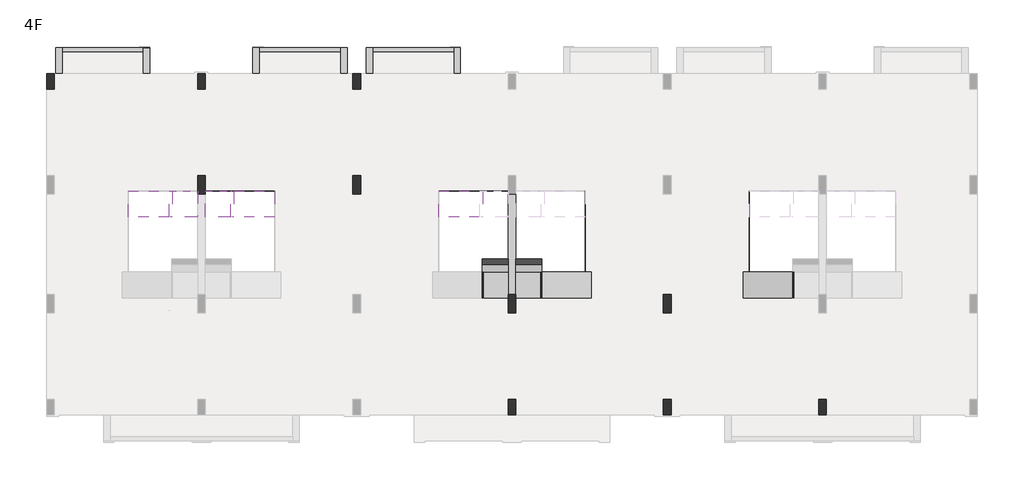
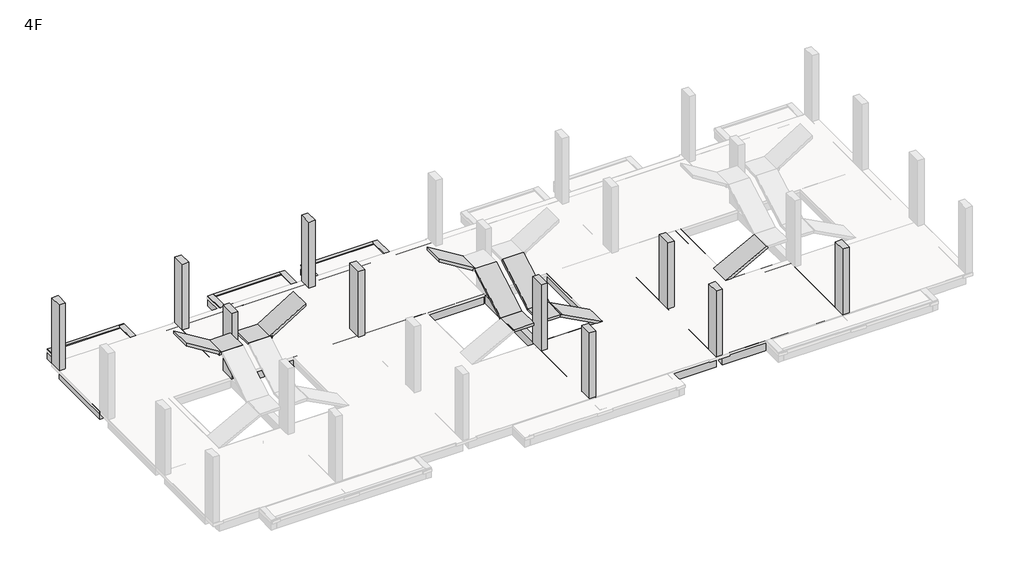
# One storey, part 2 of 3: 39 beams, 10 columns.
"""IFC4 building model written with IfcOpenShell, lengths in millimetres."""

from ifc_helpers import new_model, si_unit, frame, origin, place, context, project, spatial, polyline, outline, extrude, faceted_brep, element, save

model = new_model("IFC4")

# Units and contexts
model_context = context("Model", 3, world=origin())
ifc_project = project(units=[si_unit("LENGTHUNIT", "METRE", prefix="MILLI")], contexts=[model_context])

# Site, building, storey
site = spatial("IfcSite", under=ifc_project)
building = spatial("IfcBuilding", under=site)
storey = spatial("IfcBuildingStorey", under=building, Name="4F", Elevation=10630.0)

# Beams
placement = place(None, origin())
element("IfcBeam", 1, ObjectType="M_Concrete-Rectangular Beam : 1000x120", at=placement, inside=storey, context=model_context, shape_type="Brep", body=[
    faceted_brep([(4600.0000007, 7550.0000002, 12880.0), (4600.0000007, 8550.0000002, 12880.0), (4600.0000007, 8550.0000002, 12760.0), (4600.0000007, 7550.0000002, 12760.0), (5700.0000007, 8550.0000002, 12760.0), (5700.0000007, 8550.0000002, 12880.0), (5700.0000007, 7550.0000002, 12880.0), (5700.0000007, 7609.0063595, 12775.5095719), (5700.0000007, 7581.5414925, 12760.0), (4700.0000007, 7550.0000002, 12880.0), (4700.0000007, 7581.5414925, 12760.0), (4700.0000007, 7550.0000002, 12760.0), (4700.0000007, 7609.0063595, 12775.5095719)], [[[0, 1, 2, 3]], [[4, 5, 6, 7, 8]], [[1, 0, 9, 6, 5]], [[2, 1, 5, 4]], [[3, 2, 4, 8, 10, 11]], [[0, 3, 11, 9]], [[12, 7, 6, 9]], [[7, 12, 10, 8]], [[12, 9, 11, 10]]]),
])
element("IfcBeam", 2, ObjectType="M_Concrete-Rectangular Beam : 1000x120", at=placement, inside=storey, context=model_context, shape_type="Brep", body=[
    faceted_brep([(3019.99996, 7549.9999993, 13930.0), (4715.7503089, 7549.9999993, 12880.0), (4715.7503089, 8549.9999993, 12880.0), (3019.99996, 8549.9999993, 13930.0), (4600.0000007, 8549.9999993, 12880.0), (4600.0000007, 8549.9999993, 12810.5302519), (3020.0, 8549.9999993, 13788.8582245), (4600.0000007, 7549.9999993, 12810.5302519), (3020.0, 7549.9999993, 13788.8582245), (4600.0000007, 7549.9999993, 12880.0), (4700.0000007, 7549.9999993, 12880.0)], [[[0, 1, 2, 3]], [[3, 2, 4, 5, 6]], [[5, 7, 8, 6]], [[1, 0, 8, 7, 9, 10]], [[4, 9, 7, 5]], [[9, 4, 2, 1, 10]], [[0, 3, 6, 8]]]),
])
element("IfcBeam", 3, ObjectType="M_Concrete-Rectangular Beam : 1000x120", at=placement, inside=storey, context=model_context, shape_type="Brep", body=[
    faceted_brep([(7100.0000007, 8550.0000002, 12880.0), (7100.0000007, 7550.0000002, 12880.0), (7100.0000007, 7550.0000002, 12760.0), (7100.0000007, 8550.0000002, 12760.0), (6000.0000007, 8550.0000002, 12880.0), (6000.0000007, 8550.0000002, 12760.0), (6000.0000007, 7581.5414925, 12760.0), (6000.0000007, 7609.0063595, 12775.5095719), (6000.0000007, 7550.0000002, 12880.0), (7000.0000007, 7550.0000002, 12880.0), (7000.0000007, 7550.0000002, 12760.0), (7000.0000007, 7581.5414925, 12760.0), (7000.0000007, 7609.0063595, 12775.5095719)], [[[0, 1, 2, 3]], [[4, 5, 6, 7, 8]], [[1, 0, 4, 8, 9]], [[0, 3, 5, 4]], [[3, 2, 10, 11, 6, 5]], [[2, 1, 9, 10]], [[12, 9, 8, 7]], [[12, 7, 6, 11]], [[9, 12, 11, 10]]]),
])
element("IfcBeam", 4, ObjectType="M_Concrete-Rectangular Beam : 1000x120", at=placement, inside=storey, context=model_context, shape_type="Brep", body=[
    faceted_brep([(6984.2496926, 7549.9999993, 12880.0), (8680.0000414, 7549.9999993, 13930.0), (8680.0, 8549.9999993, 13929.9999744), (6984.2496926, 8549.9999993, 12880.0), (8680.0, 8549.9999993, 13788.8582236), (7100.0000007, 8549.9999993, 12810.5302519), (7100.0000007, 8549.9999993, 12880.0), (7100.0000007, 7549.9999993, 12810.5302519), (8680.0, 7549.9999993, 13788.8582236), (7000.0000007, 7549.9999993, 12880.0), (7100.0000007, 7549.9999993, 12880.0)], [[[0, 1, 2, 3]], [[3, 2, 4, 5, 6]], [[7, 5, 4, 8]], [[1, 0, 9, 10, 7, 8]], [[10, 6, 5, 7]], [[6, 10, 9, 0, 3]], [[2, 1, 8, 4]]]),
])
element("IfcBeam", 5, ObjectType="M_Concrete-Rectangular Beam : 1000x120", at=placement, inside=storey, context=model_context, shape_type="Brep", body=[
    faceted_brep([(16700.0000058, 7550.0000002, 12880.0), (17700.0000058, 7550.0000002, 12880.0), (17700.0000058, 7609.0063595, 12775.5095719), (16700.0000058, 7609.0063595, 12775.5095719), (16700.0000058, 5424.9999998, 11680.0), (16700.0000058, 5484.0063591, 11575.5095719), (17700.0000058, 5484.0063591, 11575.5095719), (17700.0000058, 5424.9999998, 11680.0), (17700.0000058, 5524.9999998, 11598.6589219), (17700.0000058, 7581.5414925, 12760.0), (16700.0000058, 5524.9999998, 11598.6589219), (16700.0000058, 7581.5414925, 12760.0)], [[[0, 1, 2, 3]], [[4, 5, 6, 7]], [[1, 0, 4, 7]], [[2, 1, 7, 6, 8, 9]], [[3, 2, 9, 8, 6, 5, 10, 11]], [[0, 3, 11, 10, 5, 4]]]),
])
element("IfcBeam", 6, ObjectType="M_Concrete-Rectangular Beam : 1000x120", at=placement, inside=storey, context=model_context, shape_type="Brep", body=[
    faceted_brep([(15019.9999651, 7549.9999993, 13930.0), (16715.7503139, 7549.9999993, 12880.0), (16715.7503139, 8549.9999993, 12880.0), (15019.9999651, 8549.9999993, 13930.0), (16600.0000058, 8549.9999993, 12880.0), (16600.0000058, 8549.9999993, 12810.5302519), (15020.0000057, 8549.9999993, 13788.8582241), (16600.0000058, 7549.9999993, 12810.5302519), (15020.0000057, 7549.9999993, 13788.8582241), (16600.0000058, 7549.9999993, 12880.0), (16700.0000058, 7549.9999993, 12880.0)], [[[0, 1, 2, 3]], [[3, 2, 4, 5, 6]], [[5, 7, 8, 6]], [[1, 0, 8, 7, 9, 10]], [[4, 9, 7, 5]], [[9, 4, 2, 1, 10]], [[0, 3, 6, 8]]]),
])
element("IfcBeam", 7, ObjectType="M_Concrete-Rectangular Beam : 1000x120", at=placement, inside=storey, context=model_context, shape_type="Brep", body=[
    faceted_brep([(17700.0000058, 5524.9999998, 11560.0), (16700.0000058, 5524.9999998, 11560.0), (16700.0000058, 5524.9999998, 11598.6589219), (17700.0000058, 5524.9999998, 11598.6589219), (17700.0000058, 4424.9999998, 11560.0), (17700.0000058, 4424.9999998, 11680.0), (16730.4772117, 4424.9999998, 11680.0), (16787.1330628, 4424.9999998, 11574.2166623), (16760.588832, 4424.9999998, 11560.0), (17700.0000058, 5424.9999998, 11680.0), (16700.0000058, 5424.9999998, 11680.0), (16700.0000058, 4424.9999998, 11680.0), (17700.0000058, 5484.0063591, 11575.5095719), (16760.588832, 5424.9999998, 11560.0), (16700.0000058, 5424.9999998, 11560.0), (16700.0000058, 4424.9999998, 11663.6768996), (16700.0000058, 5484.0063591, 11575.5095719), (16700.0000058, 5424.9999998, 11663.6768996), (16730.4772117, 5424.9999998, 11680.0), (16787.1330628, 5424.9999998, 11574.2166623)], [[[0, 1, 2, 3]], [[4, 5, 6, 7, 8]], [[6, 5, 9, 10, 11]], [[5, 4, 0, 3, 12, 9]], [[1, 0, 4, 8, 13, 14]], [[15, 11, 10, 16, 2, 1, 14, 17]], [[6, 18, 19, 7]], [[18, 6, 15, 17]], [[7, 19, 13, 8]], [[19, 18, 17, 14, 13]], [[11, 15, 6]], [[12, 16, 10, 9]], [[16, 12, 3, 2]]]),
])
element("IfcBeam", 8, ObjectType="M_Concrete-Rectangular Beam : 1000x120", at=placement, inside=storey, context=model_context, shape_type="Brep", body=[
    faceted_brep([(18969.5227998, 4424.9999998, 11680.0), (18969.5227998, 5424.9999998, 11680.0), (18912.8669488, 5424.9999998, 11574.2166623), (18912.8669488, 4424.9999998, 11574.2166623), (19000.0000058, 4424.9999998, 11663.6768996), (20930.0000065, 4424.9999998, 10630.0), (20930.0000065, 5424.9999998, 10630.0), (19000.0000058, 5424.9999998, 11663.6768996), (18939.4111796, 4424.9999998, 11560.0), (20675.8338483, 4424.9999998, 10630.0), (18939.4111796, 5424.9999998, 11560.0), (20680.0000058, 5424.9999998, 10627.7686732), (20680.0000058, 4449.9999998, 10627.7686732), (20675.8338483, 4449.9999998, 10630.0), (20680.0000058, 5424.9999998, 10630.0), (20680.0000058, 4449.9999998, 10630.0)], [[[0, 1, 2, 3]], [[1, 0, 4, 5, 6, 7]], [[0, 3, 8, 9, 5, 4]], [[3, 2, 10, 11, 12, 13, 9, 8]], [[2, 1, 7, 6, 14, 11, 10]], [[9, 13, 15, 14, 6, 5]], [[11, 14, 15, 12]], [[15, 13, 12]]]),
])
element("IfcBeam", 9, ObjectType="M_Concrete-Rectangular Beam : 1000x120", at=placement, inside=storey, context=model_context, shape_type="Brep", body=[
    faceted_brep([(19000.0000058, 7550.0000002, 12880.0), (19000.0000058, 7609.0063595, 12775.5095719), (18000.0000058, 7609.0063595, 12775.5095719), (18000.0000058, 7550.0000002, 12880.0), (19000.0000058, 5424.9999998, 11680.0), (18000.0000058, 5424.9999998, 11680.0), (18000.0000058, 5484.0063591, 11575.5095719), (19000.0000058, 5484.0063591, 11575.5095719), (18000.0000058, 7581.5414925, 12760.0), (18000.0000058, 5524.9999998, 11598.6589219), (19000.0000058, 7581.5414925, 12760.0), (19000.0000058, 5524.9999998, 11598.6589219)], [[[0, 1, 2, 3]], [[4, 5, 6, 7]], [[3, 5, 4, 0]], [[2, 8, 9, 6, 5, 3]], [[1, 10, 11, 7, 6, 9, 8, 2]], [[0, 4, 7, 11, 10, 1]]]),
])
element("IfcBeam", 10, ObjectType="M_Concrete-Rectangular Beam : 1000x120", at=placement, inside=storey, context=model_context, shape_type="Brep", body=[
    faceted_brep([(19000.0000058, 5524.9999998, 11560.0), (18000.0000058, 5524.9999998, 11560.0), (18000.0000058, 5524.9999998, 11598.6589219), (19000.0000058, 5524.9999998, 11598.6589219), (18000.0000058, 4424.9999998, 11680.0), (18000.0000058, 4424.9999998, 11560.0), (18939.4111796, 4424.9999998, 11560.0), (18912.8669488, 4424.9999998, 11574.2166623), (18969.5227998, 4424.9999998, 11680.0), (19000.0000058, 4424.9999998, 11680.0), (19000.0000058, 5424.9999998, 11680.0), (18000.0000058, 5424.9999998, 11680.0), (18000.0000058, 5484.0063591, 11575.5095719), (19000.0000058, 5424.9999998, 11560.0), (18939.4111796, 5424.9999998, 11560.0), (19000.0000058, 4424.9999998, 11663.6768996), (19000.0000058, 5424.9999998, 11663.6768996), (19000.0000058, 5484.0063591, 11575.5095719), (18969.5227998, 5424.9999998, 11680.0), (18912.8669488, 5424.9999998, 11574.2166623)], [[[0, 1, 2, 3]], [[4, 5, 6, 7, 8]], [[8, 9, 10, 11, 4]], [[5, 4, 11, 12, 2, 1]], [[1, 0, 13, 14, 6, 5]], [[9, 15, 16, 13, 0, 3, 17, 10]], [[18, 8, 7, 19]], [[8, 18, 16, 15]], [[19, 7, 6, 14]], [[18, 19, 14, 13, 16]], [[15, 9, 8]], [[17, 12, 11, 10]], [[12, 17, 3, 2]]]),
])
element("IfcBeam", 11, ObjectType="M_Concrete-Rectangular Beam : 1000x120", at=placement, inside=storey, context=model_context, shape_type="Brep", body=[
    faceted_brep([(28730.4772098, 5424.9999998, 11680.0), (28730.4772098, 4424.9999998, 11680.0), (28787.1330609, 4424.9999998, 11574.2166623), (28787.1330609, 5424.9999998, 11574.2166623), (28700.0000039, 5424.9999998, 11663.6768996), (26770.0000031, 5424.9999998, 10630.0), (26770.0000031, 4424.9999998, 10630.0), (28700.0000039, 4424.9999998, 11663.6768996), (27024.1661613, 4424.9999998, 10630.0), (28760.5888301, 4424.9999998, 11560.0), (27024.1661613, 4449.9999998, 10630.0), (27020.000004, 4449.9999998, 10627.7686733), (27020.000004, 5424.9999998, 10627.7686733), (28760.5888301, 5424.9999998, 11560.0), (27020.000004, 5424.9999998, 10630.0), (27020.000004, 4449.9999998, 10630.0)], [[[0, 1, 2, 3]], [[1, 0, 4, 5, 6, 7]], [[2, 1, 7, 6, 8, 9]], [[3, 2, 9, 8, 10, 11, 12, 13]], [[0, 3, 13, 12, 14, 5, 4]], [[5, 14, 15, 10, 8, 6]], [[14, 12, 11, 15]], [[10, 15, 11]]]),
])
element("IfcBeam", 12, ObjectType="M_Concrete-Rectangular Beam : 150x500", at=placement, inside=storey, context=model_context, shape_type="SweptSolid", body=[
    extrude(outline(polyline([(11225.0000398, 14100.0000002), (11225.0000398, 13950.0000002), (8090.0434249, 13950.0000002), (8090.0434249, 14100.0000002), (11225.0000398, 14100.0000002)])), frame((0.0, 0.0, 10130.0), z_axis=(0.0, 0.0, 1.0), x_axis=(1.0, 0.0, 0.0)), (0.0, 0.0, 1.0), 500.0),
])
element("IfcBeam", 13, ObjectType="M_Concrete-Rectangular Beam : 150x500", at=placement, inside=storey, context=model_context, shape_type="SweptSolid", body=[
    extrude(outline(polyline([(3609.9999642, 14075.0000066), (3609.9999642, 13950.0000002), (475.0000398, 13950.0000002), (475.0000398, 14100.0000002), (3859.9999642, 14100.0000002), (3859.9999642, 14075.0000066), (3609.9999642, 14075.0000066)])), frame((0.0, 0.0, 10130.0), z_axis=(0.0, 0.0, 1.0), x_axis=(1.0, 0.0, 0.0)), (0.0, 0.0, 1.0), 500.0),
])
element("IfcBeam", 14, ObjectType="M_Concrete-Rectangular Beam : 150x500", at=placement, inside=storey, context=model_context, shape_type="SweptSolid", body=[
    extrude(outline(polyline([(15609.727107, 14100.0000002), (15609.727107, 13950.0000002), (12475.0998336, 13950.0000002), (12475.0998336, 14100.0000002), (15609.727107, 14100.0000002)])), frame((0.0, 0.0, 10130.0), z_axis=(0.0, 0.0, 1.0), x_axis=(1.0, 0.0, 0.0)), (0.0, 0.0, 1.0), 500.0),
])
element("IfcBeam", 15, ObjectType="M_Concrete-Rectangular Beam : 250x400", at=placement, inside=storey, context=model_context, shape_type="Brep", body=[
    faceted_brep([(20930.0000058, 8549.9999993, 10630.0), (20680.0000058, 8549.9999993, 10630.0), (20680.0000058, 5424.9999998, 10630.0), (20680.0000058, 4449.9999998, 10630.0), (20930.0000058, 4449.9999998, 10630.0), (20680.0000058, 8549.9999993, 10488.8582241), (20680.0000058, 8549.9999993, 10230.0), (20680.0000058, 4449.9999998, 10230.0), (20680.0000058, 4449.9999998, 10627.7686732), (20930.0000058, 8549.9999993, 10230.0), (20930.0000058, 4449.9999998, 10230.0)], [[[0, 1, 2, 3, 4]], [[1, 5, 6, 7, 8, 3, 2]], [[6, 9, 10, 7]], [[9, 0, 4, 10]], [[1, 0, 9, 6, 5]], [[4, 3, 8, 7, 10]]]),
])
element("IfcBeam", 16, ObjectType="M_Concrete-Rectangular Beam : 250x400", at=placement, inside=storey, context=model_context, shape_type="Brep", body=[
    faceted_brep([(27020.000004, 8549.9999993, 10630.0), (26770.000004, 8549.9999993, 10630.0), (26770.000004, 4449.9999998, 10630.0), (27020.000004, 4449.9999998, 10630.0), (27020.000004, 5424.9999998, 10630.0), (27020.000004, 8549.9999993, 10230.0), (27020.000004, 8549.9999993, 10488.8582239), (27020.000004, 4449.9999998, 10627.7686733), (27020.000004, 4449.9999998, 10230.0), (26770.000004, 8549.9999993, 10230.0), (26770.000004, 4449.9999998, 10230.0)], [[[0, 1, 2, 3, 4]], [[5, 6, 0, 4, 3, 7, 8]], [[9, 5, 8, 10]], [[1, 9, 10, 2]], [[1, 0, 6, 5, 9]], [[3, 2, 10, 8, 7]]]),
])
element("IfcBeam", 17, ObjectType="M_Concrete-Rectangular Beam : 250x500", at=placement, inside=storey, context=model_context, shape_type="Brep", body=[
    faceted_brep([(225.0000398, 13101.5853605, 10630.0), (225.0000398, 13101.5853605, 10130.0), (475.0000398, 13101.5853605, 10130.0), (475.0000398, 13101.5853605, 10630.0), (475.0000398, 13950.0000002, 10630.0), (475.0000398, 14100.0000002, 10630.0), (225.0000398, 14100.0000002, 10630.0), (475.0000398, 13950.0000002, 10130.0), (475.0000398, 14100.0000002, 10130.0), (225.0000398, 14100.0000002, 10130.0)], [[[0, 1, 2, 3]], [[0, 3, 4, 5, 6]], [[3, 2, 7, 8, 5, 4]], [[2, 1, 9, 8, 7]], [[1, 0, 6, 9]], [[6, 5, 8, 9]]]),
])
element("IfcBeam", 18, ObjectType="M_Concrete-Rectangular Beam : 250x500", at=placement, inside=storey, context=model_context, shape_type="Brep", body=[
    faceted_brep([(11475.0000398, 14100.0000002, 10630.0), (11225.0000398, 14100.0000002, 10630.0), (11225.0000398, 13950.0000002, 10630.0), (11225.0000398, 13100.0000001, 10630.0), (11475.0000398, 13100.0000001, 10630.0), (11225.0000398, 14100.0000002, 10130.0), (11225.0000398, 13950.0000002, 10130.0), (11225.0000398, 13100.0000001, 10130.0), (11475.0000398, 14100.0000002, 10130.0), (11475.0000398, 13100.0000001, 10130.0)], [[[0, 1, 2, 3, 4]], [[1, 5, 6, 7, 3, 2]], [[5, 8, 9, 7, 6]], [[8, 0, 4, 9]], [[1, 0, 8, 5]], [[4, 3, 7, 9]]]),
])
element("IfcBeam", 19, ObjectType="M_Concrete-Rectangular Beam : 250x500", at=placement, inside=storey, context=model_context, shape_type="Brep", body=[
    faceted_brep([(8090.0434249, 14100.0000002, 10630.0), (8090.0434249, 14100.0000002, 10130.0), (7840.0434249, 14100.0000002, 10130.0), (7840.0434249, 14100.0000002, 10630.0), (7840.0434249, 13100.0000001, 10630.0), (8090.0434249, 13100.0000001, 10630.0), (8090.0434249, 13950.0000002, 10630.0), (7840.0434249, 13100.0000001, 10130.0), (8090.0434249, 13950.0000002, 10130.0), (8090.0434249, 13100.0000001, 10130.0)], [[[0, 1, 2, 3]], [[0, 3, 4, 5, 6]], [[3, 2, 7, 4]], [[2, 1, 8, 9, 7]], [[1, 0, 6, 5, 9, 8]], [[5, 4, 7, 9]]]),
])
element("IfcBeam", 20, ObjectType="M_Concrete-Rectangular Beam : 250x500", at=placement, inside=storey, context=model_context, shape_type="Brep", body=[
    faceted_brep([(3609.9999642, 14075.0000066, 10130.0), (3609.9999642, 14075.0000066, 10630.0), (3859.9999642, 14075.0000066, 10630.0), (3859.9999642, 14075.0000066, 10130.0), (3609.9999642, 13950.0000002, 10630.0), (3609.9999642, 13100.0000001, 10630.0), (3859.9999642, 13100.0000001, 10630.0), (3859.9999642, 13100.0000001, 10130.0), (3609.9999642, 13100.0000001, 10130.0), (3609.9999642, 13950.0000002, 10130.0)], [[[0, 1, 2, 3]], [[2, 1, 4, 5, 6]], [[3, 2, 6, 7]], [[0, 3, 7, 8, 9]], [[1, 0, 9, 8, 5, 4]], [[6, 5, 8, 7]]]),
])
element("IfcBeam", 21, ObjectType="M_Concrete-Rectangular Beam : 250x500", at=placement, inside=storey, context=model_context, shape_type="Brep", body=[
    faceted_brep([(12475.0998336, 14100.0000002, 10630.0), (12225.0998336, 14100.0000002, 10630.0), (12225.0998336, 13100.0000001, 10630.0), (12475.0998336, 13100.0000001, 10630.0), (12475.0998336, 13950.0000002, 10630.0), (12475.0998336, 14100.0000002, 10130.0), (12475.0998336, 13100.0000001, 10130.0), (12475.0998336, 13950.0000002, 10130.0), (12225.0998336, 14100.0000002, 10130.0), (12225.0998336, 13100.0000001, 10130.0)], [[[0, 1, 2, 3, 4]], [[5, 0, 4, 3, 6, 7]], [[8, 5, 7, 6, 9]], [[1, 8, 9, 2]], [[1, 0, 5, 8]], [[3, 2, 9, 6]]]),
])
element("IfcBeam", 22, ObjectType="M_Concrete-Rectangular Beam : 250x500", at=placement, inside=storey, context=model_context, shape_type="Brep", body=[
    faceted_brep([(15859.727107, 14100.0000002, 10630.0), (15609.727107, 14100.0000002, 10630.0), (15609.727107, 13950.0000002, 10630.0), (15609.727107, 13100.0000001, 10630.0), (15859.727107, 13100.0000001, 10630.0), (15859.727107, 14100.0000002, 10130.0), (15859.727107, 13100.0000001, 10130.0), (15609.727107, 14100.0000002, 10130.0), (15609.727107, 13100.0000001, 10130.0), (15609.727107, 13950.0000002, 10130.0)], [[[0, 1, 2, 3, 4]], [[5, 0, 4, 6]], [[7, 5, 6, 8, 9]], [[1, 7, 9, 8, 3, 2]], [[4, 3, 8, 6]], [[1, 0, 5, 7]]]),
])
element("IfcBeam", 23, ObjectType="M_Concrete-Rectangular Beam : 300x400", at=placement, inside=storey, context=model_context, shape_type="SweptSolid", body=[
    extrude(outline(polyline([(165.0, 9150.0000002), (-135.0, 9150.0000002), (-135.0, 12500.0000005), (165.0, 12500.0000005), (165.0, 9150.0000002)])), frame((0.0, 0.0, 10230.0), z_axis=(0.0, 0.0, 1.0), x_axis=(1.0, 0.0, 0.0)), (0.0, 0.0, 1.0), 400.0),
])
element("IfcBeam", 24, ObjectType="M_Concrete-Rectangular Beam : 300x400", at=placement, inside=storey, context=model_context, shape_type="SweptSolid", body=[
    extrude(outline(polyline([(18000.0000046, 4550.0000002), (17700.0000046, 4550.0000002), (17700.0000046, 8450.0000002), (18000.0000046, 8450.0000002), (18000.0000046, 4550.0000002)])), frame((0.0, 0.0, 10230.0), z_axis=(0.0, 0.0, 1.0), x_axis=(1.0, 0.0, 0.0)), (0.0, 0.0, 1.0), 400.0),
])
element("IfcBeam", 25, ObjectType="M_Concrete-Rectangular Beam : 300x400", at=placement, inside=storey, context=model_context, shape_type="SweptSolid", body=[
    extrude(outline(polyline([(18000.0000046, 500.0), (17700.0000046, 500.0), (17700.0000046, 3850.0000002), (18000.0000046, 3850.0000002), (18000.0000046, 500.0)])), frame((0.0, 0.0, 10230.0), z_axis=(0.0, 0.0, 1.0), x_axis=(1.0, 0.0, 0.0)), (0.0, 0.0, 1.0), 400.0),
])
element("IfcBeam", 26, ObjectType="M_Concrete-Rectangular Beam : 300x400", at=placement, inside=storey, context=model_context, shape_type="SweptSolid", body=[
    extrude(outline(polyline([(30000.0000031, 500.0), (29700.0000031, 500.0), (29700.0000031, 3850.0000002), (30000.0000031, 3850.0000002), (30000.0000031, 500.0)])), frame((0.0, 0.0, 10230.0), z_axis=(0.0, 0.0, 1.0), x_axis=(1.0, 0.0, 0.0)), (0.0, 0.0, 1.0), 400.0),
])
element("IfcBeam", 27, ObjectType="M_Concrete-Rectangular Beam : 300x400", at=placement, inside=storey, context=model_context, shape_type="SweptSolid", body=[
    extrude(outline(polyline([(24000.000004, 500.0), (23700.000004, 500.0), (23700.000004, 3850.0000002), (24000.000004, 3850.0000002), (24000.000004, 500.0)])), frame((0.0, 0.0, 10230.0), z_axis=(0.0, 0.0, 1.0), x_axis=(1.0, 0.0, 0.0)), (0.0, 0.0, 1.0), 400.0),
])
element("IfcBeam", 28, ObjectType="M_Concrete-Rectangular Beam : 300x400", at=placement, inside=storey, context=model_context, shape_type="SweptSolid", body=[
    extrude(outline(polyline([(24000.000004, 4550.0000002), (23700.000004, 4550.0000002), (23700.000004, 8450.0000002), (24000.000004, 8450.0000002), (24000.000004, 4550.0000002)])), frame((0.0, 0.0, 10230.0), z_axis=(0.0, 0.0, 1.0), x_axis=(1.0, 0.0, 0.0)), (0.0, 0.0, 1.0), 400.0),
])
element("IfcBeam", 29, ObjectType="M_Concrete-Rectangular Beam : 300x400", at=placement, inside=storey, context=model_context, shape_type="SweptSolid", body=[
    extrude(outline(polyline([(6000.0000007, 9150.0000002), (5700.0000007, 9150.0000002), (5700.0000007, 12500.0000005), (6000.0000007, 12500.0000005), (6000.0000007, 9150.0000002)])), frame((0.0, 0.0, 10230.0), z_axis=(0.0, 0.0, 1.0), x_axis=(1.0, 0.0, 0.0)), (0.0, 0.0, 1.0), 400.0),
])
element("IfcBeam", 30, ObjectType="M_Concrete-Rectangular Beam : 300x400", at=placement, inside=storey, context=model_context, shape_type="SweptSolid", body=[
    extrude(outline(polyline([(12000.0000034, 9150.0000002), (11700.0000034, 9150.0000002), (11700.0000034, 12500.0000005), (12000.0000034, 12500.0000005), (12000.0000034, 9150.0000002)])), frame((0.0, 0.0, 10230.0), z_axis=(0.0, 0.0, 1.0), x_axis=(1.0, 0.0, 0.0)), (0.0, 0.0, 1.0), 400.0),
])
element("IfcBeam", 31, ObjectType="M_Concrete-Rectangular Beam : 300x500", at=placement, inside=storey, context=model_context, shape_type="Brep", body=[
    faceted_brep([(164.9999993, 13100.0000001, 10630.0), (164.9999993, 12800.0000001, 10630.0), (5700.0000007, 12800.0000001, 10630.0), (5700.0000007, 13100.0000001, 10630.0), (3859.9999642, 13100.0000001, 10630.0), (3609.9999642, 13100.0000001, 10630.0), (164.9999993, 12800.0000001, 10130.0), (5700.0000007, 12800.0000001, 10130.0), (164.9999993, 13100.0000001, 10130.0), (3609.9999642, 13100.0000001, 10130.0), (3859.9999642, 13100.0000001, 10130.0), (5700.0000007, 13100.0000001, 10130.0)], [[[0, 1, 2, 3, 4, 5]], [[1, 6, 7, 2]], [[6, 8, 9, 10, 11, 7]], [[8, 0, 5, 4, 3, 11, 10, 9]], [[1, 0, 8, 6]], [[3, 2, 7, 11]]]),
])
element("IfcBeam", 32, ObjectType="M_Concrete-Rectangular Beam : 300x500", at=placement, inside=storey, context=model_context, shape_type="Brep", body=[
    faceted_brep([(6000.0000007, 13100.0000001, 10630.0), (6000.0000007, 12800.0000001, 10630.0), (11700.0000034, 12800.0000001, 10630.0), (11700.0000034, 13100.0000001, 10630.0), (11475.0000398, 13100.0000001, 10630.0), (11225.0000398, 13100.0000001, 10630.0), (8090.0434249, 13100.0000001, 10630.0), (7840.0434249, 13100.0000001, 10630.0), (6000.0000007, 12800.0000001, 10130.0), (11700.0000034, 12800.0000001, 10130.0), (6000.0000007, 13100.0000001, 10130.0), (7840.0434249, 13100.0000001, 10130.0), (8090.0434249, 13100.0000001, 10130.0), (11225.0000398, 13100.0000001, 10130.0), (11475.0000398, 13100.0000001, 10130.0), (11700.0000034, 13100.0000001, 10130.0)], [[[0, 1, 2, 3, 4, 5, 6, 7]], [[1, 8, 9, 2]], [[8, 10, 11, 12, 13, 14, 15, 9]], [[10, 0, 7, 6, 5, 4, 3, 15, 14, 13, 12, 11]], [[1, 0, 10, 8]], [[3, 2, 9, 15]]]),
])
element("IfcBeam", 33, ObjectType="M_Concrete-Rectangular Beam : 300x500", at=placement, inside=storey, context=model_context, shape_type="Brep", body=[
    faceted_brep([(5999.9649933, 8849.9999993, 10630.0), (5999.9649933, 8549.9999993, 10630.0), (8680.0, 8549.9999993, 10630.0), (8930.0, 8549.9999993, 10630.0), (11699.964996, 8549.9999993, 10630.0), (11699.964996, 8849.9999993, 10630.0), (5999.9649933, 8549.9999993, 10130.0), (11699.964996, 8549.9999993, 10130.0), (5999.9649933, 8849.9999993, 10130.0), (11699.964996, 8849.9999993, 10130.0)], [[[0, 1, 2, 3, 4, 5]], [[1, 6, 7, 4, 3, 2]], [[6, 8, 9, 7]], [[8, 0, 5, 9]], [[1, 0, 8, 6]], [[5, 4, 7, 9]]]),
])
element("IfcBeam", 34, ObjectType="M_Concrete-Rectangular Beam : 300x500", at=placement, inside=storey, context=model_context, shape_type="Brep", body=[
    faceted_brep([(12000.0000034, 13100.0000001, 10630.0), (12000.0000034, 12800.0000001, 10630.0), (17700.0000058, 12800.0000001, 10630.0), (17700.0000058, 13100.0000001, 10630.0), (15859.727107, 13100.0000001, 10630.0), (15609.727107, 13100.0000001, 10630.0), (12475.0998336, 13100.0000001, 10630.0), (12225.0998336, 13100.0000001, 10630.0), (12000.0000034, 12800.0000001, 10130.0), (17700.0000058, 12800.0000001, 10130.0), (12000.0000034, 13100.0000001, 10130.0), (12225.0998336, 13100.0000001, 10130.0), (12475.0998336, 13100.0000001, 10130.0), (15609.727107, 13100.0000001, 10130.0), (15859.727107, 13100.0000001, 10130.0), (17700.0000058, 13100.0000001, 10130.0)], [[[0, 1, 2, 3, 4, 5, 6, 7]], [[1, 8, 9, 2]], [[8, 10, 11, 12, 13, 14, 15, 9]], [[10, 0, 7, 6, 5, 4, 3, 15, 14, 13, 12, 11]], [[10, 8, 1, 0]], [[3, 2, 9, 15]]]),
])
element("IfcBeam", 35, ObjectType="M_Concrete-Rectangular Beam : 300x500", at=placement, inside=storey, context=model_context, shape_type="Brep", body=[
    faceted_brep([(11999.964996, 8849.9999993, 10630.0), (12000.0000027, 8549.9999993, 10630.0), (14770.0000057, 8549.9999993, 10630.0), (15020.0000057, 8549.9999993, 10630.0), (17699.9649983, 8549.9999993, 10630.0), (17699.9649983, 8849.9999993, 10630.0), (11999.964996, 8549.9999993, 10130.0), (17699.9649983, 8549.9999993, 10130.0), (11999.964996, 8849.9999993, 10130.0), (17699.9649983, 8849.9999993, 10130.0)], [[[0, 1, 2, 3, 4, 5]], [[1, 6, 7, 4, 3, 2]], [[6, 8, 9, 7]], [[8, 0, 5, 9]], [[8, 6, 1, 0]], [[5, 4, 7, 9]]]),
])
element("IfcBeam", 36, ObjectType="M_Concrete-Rectangular Beam : 300x500", at=placement, inside=storey, context=model_context, shape_type="Brep", body=[
    faceted_brep([(18000.0000058, 4449.9999998, 10630.0), (18000.0000058, 4149.9999998, 10630.0), (23700.0000047, 4149.9999998, 10630.0), (23700.0000047, 4449.9999998, 10630.0), (20930.0000058, 4449.9999998, 10630.0), (20680.0000058, 4449.9999998, 10630.0), (20675.8338483, 4449.9999998, 10630.0), (18000.0000058, 4149.9999998, 10130.0), (23700.0000047, 4149.9999998, 10130.0), (18000.0000058, 4449.9999998, 10130.0), (23700.0000047, 4449.9999998, 10130.0)], [[[0, 1, 2, 3, 4, 5, 6]], [[1, 7, 8, 2]], [[7, 9, 10, 8]], [[9, 0, 6, 5, 4, 3, 10]], [[1, 0, 9, 7]], [[3, 2, 8, 10]]]),
])
element("IfcBeam", 37, ObjectType="M_Concrete-Rectangular Beam : 300x500", at=placement, inside=storey, context=model_context, shape_type="SweptSolid", body=[
    extrude(outline(polyline([(18000.0000058, -100.0000007), (18000.0000058, 199.9999993), (23700.0000047, 199.9999993), (23700.0000047, -100.0000007), (18000.0000058, -100.0000007)])), frame((0.0, 0.0, 10130.0), z_axis=(0.0, 0.0, 1.0), x_axis=(1.0, 0.0, 0.0)), (0.0, 0.0, 1.0), 500.0),
])
element("IfcBeam", 38, ObjectType="M_Concrete-Rectangular Beam : 300x500", at=placement, inside=storey, context=model_context, shape_type="Brep", body=[
    faceted_brep([(24000.0000047, 4449.9999998, 10630.0), (24000.000004, 4149.9999998, 10630.0), (29700.0000039, 4149.9999998, 10630.0), (29700.0000039, 4449.9999998, 10630.0), (27024.1661613, 4449.9999998, 10630.0), (27020.000004, 4449.9999998, 10630.0), (26770.000004, 4449.9999998, 10630.0), (24000.0000047, 4149.9999998, 10130.0), (29700.0000039, 4149.9999998, 10130.0), (24000.0000047, 4449.9999998, 10130.0), (29700.0000039, 4449.9999998, 10130.0)], [[[0, 1, 2, 3, 4, 5, 6]], [[1, 7, 8, 2]], [[7, 9, 10, 8]], [[9, 0, 6, 5, 4, 3, 10]], [[9, 7, 1, 0]], [[3, 2, 8, 10]]]),
])
element("IfcBeam", 39, ObjectType="M_Concrete-Rectangular Beam : 300x500", at=placement, inside=storey, context=model_context, shape_type="Brep", body=[
    faceted_brep([(24000.000004, 199.9999987, 10630.0), (24000.0000047, -100.0000013, 10630.0), (26070.012858, -100.0000013, 10630.0), (26320.012858, -100.0000013, 10630.0), (29700.0000039, -100.0000013, 10630.0), (29700.0000039, 199.9999987, 10630.0), (24000.0000047, -100.0000013, 10130.0), (26070.012858, -100.0000013, 10130.0), (26320.012858, -100.0000013, 10130.0), (29700.0000039, -100.0000013, 10130.0), (24000.0000047, 199.9999987, 10130.0), (29700.0000039, 199.9999987, 10130.0)], [[[0, 1, 2, 3, 4, 5]], [[1, 6, 7, 8, 9, 4, 3, 2]], [[6, 10, 11, 9, 8, 7]], [[10, 0, 5, 11]], [[6, 1, 0, 10]], [[5, 4, 9, 11]]]),
])

# Columns
element("IfcColumn", 40, ObjectType="M_Concrete-Rectangular-Column : 300x600", at=placement, inside=storey, context=model_context, shape_type="SweptSolid", body=[
    extrude(outline(polyline([(164.9999993, 13100.0000005), (164.9999993, 12500.0000005), (-135.0000007, 12500.0000005), (-135.0000007, 13100.0000005), (164.9999993, 13100.0000005)])), frame((0.0, 0.0, 10630.0), z_axis=(0.0, 0.0, 1.0), x_axis=(1.0, 0.0, 0.0)), (0.0, 0.0, 1.0), 3300.0),
])
element("IfcColumn", 41, ObjectType="M_Concrete-Rectangular-Column : 300x600", at=placement, inside=storey, context=model_context, shape_type="SweptSolid", body=[
    extrude(outline(polyline([(18000.0000058, 500.0), (18000.0000058, -100.0), (17700.0000058, -100.0), (17700.0000058, 500.0), (18000.0000058, 500.0)])), frame((0.0, 0.0, 10630.0), z_axis=(0.0, 0.0, 1.0), x_axis=(1.0, 0.0, 0.0)), (0.0, 0.0, 1.0), 3300.0),
])
element("IfcColumn", 42, ObjectType="M_Concrete-Rectangular-Column : 300x600", at=placement, inside=storey, context=model_context, shape_type="SweptSolid", body=[
    extrude(outline(polyline([(24000.0000047, 500.0), (24000.0000047, -100.0), (23700.0000047, -100.0), (23700.0000047, 500.0), (24000.0000047, 500.0)])), frame((0.0, 0.0, 10630.0), z_axis=(0.0, 0.0, 1.0), x_axis=(1.0, 0.0, 0.0)), (0.0, 0.0, 1.0), 3300.0),
])
element("IfcColumn", 43, ObjectType="M_Concrete-Rectangular-Column : 300x600", at=placement, inside=storey, context=model_context, shape_type="SweptSolid", body=[
    extrude(outline(polyline([(6000.0000007, 13100.0000005), (6000.0000007, 12500.0000005), (5700.0000007, 12500.0000005), (5700.0000007, 13100.0000005), (6000.0000007, 13100.0000005)])), frame((0.0, 0.0, 10630.0), z_axis=(0.0, 0.0, 1.0), x_axis=(1.0, 0.0, 0.0)), (0.0, 0.0, 1.0), 3300.0),
])
element("IfcColumn", 44, ObjectType="M_Concrete-Rectangular-Column : 300x600", at=placement, inside=storey, context=model_context, shape_type="SweptSolid", body=[
    extrude(outline(polyline([(12000.0000034, 13100.0000005), (12000.0000034, 12500.0000005), (11700.0000034, 12500.0000005), (11700.0000034, 13100.0000005), (12000.0000034, 13100.0000005)])), frame((0.0, 0.0, 10630.0), z_axis=(0.0, 0.0, 1.0), x_axis=(1.0, 0.0, 0.0)), (0.0, 0.0, 1.0), 3300.0),
])
element("IfcColumn", 45, ObjectType="M_Concrete-Rectangular-Column : 300x600", at=placement, inside=storey, context=model_context, shape_type="SweptSolid", body=[
    extrude(outline(polyline([(30000.0000039, 500.0), (30000.0000039, -100.0), (29700.0000039, -100.0), (29700.0000039, 500.0), (30000.0000039, 500.0)])), frame((0.0, 0.0, 10630.0), z_axis=(0.0, 0.0, 1.0), x_axis=(1.0, 0.0, 0.0)), (0.0, 0.0, 1.0), 3300.0),
])
element("IfcColumn", 46, ObjectType="M_Concrete-Rectangular-Column : 300x700", at=placement, inside=storey, context=model_context, shape_type="SweptSolid", body=[
    extrude(outline(polyline([(18000.0000058, 4550.0000002), (18000.0000058, 3850.0000002), (17700.0000058, 3850.0000002), (17700.0000058, 4550.0000002), (18000.0000058, 4550.0000002)])), frame((0.0, 0.0, 10630.0), z_axis=(0.0, 0.0, 1.0), x_axis=(1.0, 0.0, 0.0)), (0.0, 0.0, 1.0), 3300.0),
])
element("IfcColumn", 47, ObjectType="M_Concrete-Rectangular-Column : 300x700", at=placement, inside=storey, context=model_context, shape_type="SweptSolid", body=[
    extrude(outline(polyline([(24000.0000047, 4550.0000002), (24000.0000047, 3850.0000002), (23700.0000047, 3850.0000002), (23700.0000047, 4550.0000002), (24000.0000047, 4550.0000002)])), frame((0.0, 0.0, 10630.0), z_axis=(0.0, 0.0, 1.0), x_axis=(1.0, 0.0, 0.0)), (0.0, 0.0, 1.0), 3300.0),
])
element("IfcColumn", 48, ObjectType="M_Concrete-Rectangular-Column : 300x700", at=placement, inside=storey, context=model_context, shape_type="SweptSolid", body=[
    extrude(outline(polyline([(5999.9649933, 9150.0000002), (5999.9649933, 8450.0000002), (5699.9649933, 8450.0000002), (5699.9649933, 9150.0000002), (5999.9649933, 9150.0000002)])), frame((0.0, 0.0, 10630.0), z_axis=(0.0, 0.0, 1.0), x_axis=(1.0, 0.0, 0.0)), (0.0, 0.0, 1.0), 3300.0),
])
element("IfcColumn", 49, ObjectType="M_Concrete-Rectangular-Column : 300x700", at=placement, inside=storey, context=model_context, shape_type="SweptSolid", body=[
    extrude(outline(polyline([(11999.964996, 9150.0000002), (11999.964996, 8450.0000002), (11699.964996, 8450.0000002), (11699.964996, 9150.0000002), (11999.964996, 9150.0000002)])), frame((0.0, 0.0, 10630.0), z_axis=(0.0, 0.0, 1.0), x_axis=(1.0, 0.0, 0.0)), (0.0, 0.0, 1.0), 3300.0),
])

save(model, "model.ifc")

# Revit data of these elements
# Type "M_Concrete-Rectangular Beam : 1000x120"
#   Length [instance default] = 1524 mm
#   b = 1000 mm
#   h = 120 mm
#   Structural Material [instance default] = Concrete, Cast-in-Place gray
#   Assembly Code = ""
# Type "M_Concrete-Rectangular Beam : 150x500"
#   Length [instance default] = 1524 mm
#   b = 150 mm
#   h = 500 mm
#   Structural Material [instance default] = Concrete, Cast-in-Place gray
#   Assembly Code = ""
# Type "M_Concrete-Rectangular Beam : 250x400"
#   Length [instance default] = 1524 mm
#   b = 250 mm
#   h = 400 mm
#   Structural Material [instance default] = Concrete, Cast-in-Place gray
#   Assembly Code = ""
# Type "M_Concrete-Rectangular Beam : 250x500"
#   Length [instance default] = 1524 mm
#   b = 250 mm
#   h = 500 mm
#   Structural Material [instance default] = Concrete, Cast-in-Place gray
#   Assembly Code = ""
# Type "M_Concrete-Rectangular Beam : 300x400"
#   Length [instance default] = 1524 mm
#   b = 300 mm
#   h = 400 mm
#   Structural Material [instance default] = Concrete, Cast-in-Place gray
#   Assembly Code = ""
# Type "M_Concrete-Rectangular Beam : 300x500"
#   Length [instance default] = 1524 mm
#   b = 300 mm
#   h = 500 mm
#   Structural Material [instance default] = Concrete, Cast-in-Place gray
#   Assembly Code = ""
# Type "M_Concrete-Rectangular-Column : 300x600"
#   b = 300 mm
#   h = 600 mm
#   Structural Material [instance default] = Concrete, Cast-in-Place gray
# Type "M_Concrete-Rectangular-Column : 300x700"
#   b = 300 mm
#   h = 700 mm
#   Structural Material [instance default] = Concrete, Cast-in-Place gray
# Elements 1, 2, 3, 4, 5, 6, 7, 9, 10 (IfcBeam, "M_Concrete-Rectangular Beam : 1000x120")
#   COF_GEN__Name = "STAIR"
#   Structural Material = Concrete, Cast-in-Place gray
#   Phase Created = New Construction
#   Materials on its faces: "Concrete, Cast-in-Place gray"
# Elements 8, 11 (IfcBeam, "M_Concrete-Rectangular Beam : 1000x120")
#   Comments = ""
#   COF_GEN__Name = "STAIR"
#   Structural Material = Concrete, Cast-in-Place gray
#   Phase Created = New Construction
#   Materials on its faces: "Concrete, Cast-in-Place gray"
# Elements 12, 14 (IfcBeam, "M_Concrete-Rectangular Beam : 150x500")
#   Comments = ""
#   COF_CON__WorkItemNumber = "SH3-A-03F"
#   COF_GEN__Name = "DP5"
#   Structural Material = Concrete, Cast-in-Place gray
#   Phase Created = New Construction
#   Materials on its faces: "Concrete, Cast-in-Place gray"
# Element 13 (IfcBeam, "M_Concrete-Rectangular Beam : 150x500")
#   Comments = ""
#   COF_CON__WorkItemNumber = "SH3-A-03F"
#   COF_GEN__Name = "DP5"
#   Phase Created = New Construction
#   Materials on its faces: "Concrete, Cast-in-Place gray"
# Elements 15, 16 (IfcBeam, "M_Concrete-Rectangular Beam : 250x400")
#   Comments = ""
#   COF_CON__WorkItemNumber = "SH3-A-03F"
#   COF_GEN__Name = "DP1"
#   Structural Material = Concrete, Cast-in-Place gray
#   Phase Created = New Construction
#   Materials on its faces: "Concrete, Cast-in-Place gray"
# Elements 17, 18, 21 (IfcBeam, "M_Concrete-Rectangular Beam : 250x500")
#   Comments = ""
#   COF_CON__WorkItemNumber = "SH3-A-03F"
#   COF_GEN__Name = "DP2A"
#   Structural Material = Concrete, Cast-in-Place gray
#   Phase Created = New Construction
#   Materials on its faces: "Concrete, Cast-in-Place gray"
# Elements 19, 20, 22 (IfcBeam, "M_Concrete-Rectangular Beam : 250x500")
#   Comments = ""
#   COF_GEN__Name = "DP2A"
#   Structural Material = Concrete, Cast-in-Place gray
#   Phase Created = New Construction
#   Materials on its faces: "Concrete, Cast-in-Place gray"
# Elements 23, 27, 28, 30 (IfcBeam, "M_Concrete-Rectangular Beam : 300x400")
#   Comments = ""
#   COF_CON__WorkItemNumber = "SH3-A-03F"
#   COF_GEN__Name = "D3"
#   Structural Material = Concrete, Cast-in-Place gray
#   Phase Created = New Construction
#   Materials on its faces: "Concrete, Cast-in-Place gray"
# Elements 24, 25, 26, 29 (IfcBeam, "M_Concrete-Rectangular Beam : 300x400")
#   Comments = ""
#   COF_CON__WorkItemNumber = "SH3-A-03F"
#   COF_GEN__Name = "D6"
#   Structural Material = Concrete, Cast-in-Place gray
#   Phase Created = New Construction
#   Materials on its faces: "Concrete, Cast-in-Place gray"
# Elements 31, 32, 34, 37, 39 (IfcBeam, "M_Concrete-Rectangular Beam : 300x500")
#   Comments = ""
#   COF_CON__WorkItemNumber = "SH3-A-03F"
#   COF_GEN__Name = "D1"
#   Structural Material = Concrete, Cast-in-Place gray
#   Phase Created = New Construction
#   Materials on its faces: "Concrete, Cast-in-Place gray"
# Elements 33, 35, 36, 38 (IfcBeam, "M_Concrete-Rectangular Beam : 300x500")
#   Comments = ""
#   COF_CON__WorkItemNumber = "SH3-A-03F"
#   COF_GEN__Name = "D2"
#   Structural Material = Concrete, Cast-in-Place gray
#   Phase Created = New Construction
#   Materials on its faces: "Concrete, Cast-in-Place gray"
# Elements 40, 42, 43, 44, 45 (IfcColumn, "M_Concrete-Rectangular-Column : 300x600")
#   Comments = ""
#   COF_CON__WorkItemNumber = "SH3-A-04F"
#   COF_GEN__Name = "C1"
#   Structural Material = Concrete, Cast-in-Place gray
#   Phase Created = New Construction
#   Materials on its faces: "Concrete, Cast-in-Place gray"
# Element 41 (IfcColumn, "M_Concrete-Rectangular-Column : 300x600")
#   Comments = ""
#   COF_CON__WorkItemNumber = "SH3-A-04F"
#   COF_GEN__Name = "C2"
#   Structural Material = Concrete, Cast-in-Place gray
#   Phase Created = New Construction
#   Materials on its faces: "Concrete, Cast-in-Place gray"
# Element 46 (IfcColumn, "M_Concrete-Rectangular-Column : 300x700")
#   Comments = ""
#   COF_CON__WorkItemNumber = "SH3-A-04F"
#   COF_GEN__Name = "C6"
#   Structural Material = Concrete, Cast-in-Place gray
#   Phase Created = New Construction
#   Materials on its faces: "Concrete, Cast-in-Place gray"
# Elements 47, 49 (IfcColumn, "M_Concrete-Rectangular-Column : 300x700")
#   Comments = ""
#   COF_CON__WorkItemNumber = "SH3-A-04F"
#   COF_GEN__Name = "C5"
#   Structural Material = Concrete, Cast-in-Place gray
#   Phase Created = New Construction
#   Materials on its faces: "Concrete, Cast-in-Place gray"
# Element 48 (IfcColumn, "M_Concrete-Rectangular-Column : 300x700")
#   Comments = ""
#   COF_CON__WorkItemNumber = "SH3-A-04F"
#   COF_GEN__Name = "C4"
#   Structural Material = Concrete, Cast-in-Place gray
#   Phase Created = New Construction
#   Materials on its faces: "Concrete, Cast-in-Place gray"
# Materials
#   "Concrete, Cast-in-Place gray": class "Concrete", colour RGB 207 208 204, transparency 0, Description = "Cast-in-place concrete", Cost = 0
